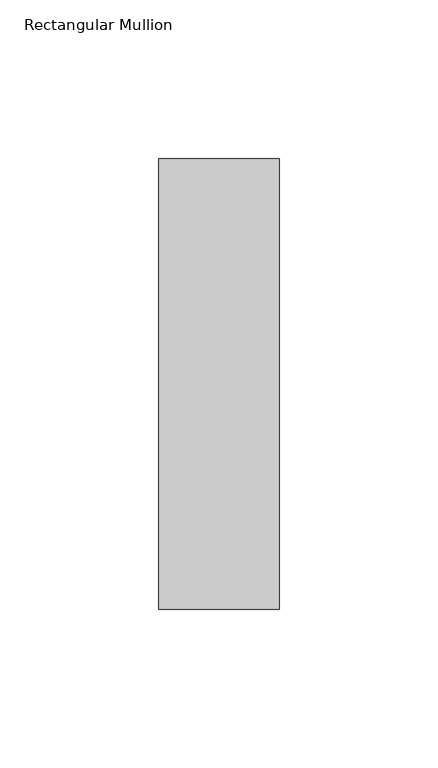
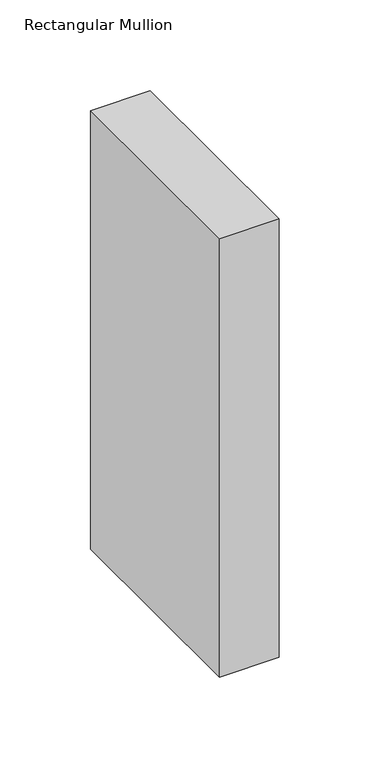
"""IFC4 building model written with IfcOpenShell, lengths in millimetres: member geometry, Rectangular Mullion : NLRS_21_CWM_hsb-regel 38x142_gen_rsf."""

from ifc_helpers import new_model, si_unit, frame, origin, place, context, project, spatial, polyline, outline, extrude, source, transform, mapped, element, save


def rectangular_mullion_e102e68a(model_context):
    return source(origin(), model_context, "Body", "SweptSolid", [
        extrude(outline(polyline([(-38.0, -71.0), (-38.0, 71.0), (0.0, 71.0), (0.0, -71.0), (-38.0, -71.0)])), frame((0.0, 0.0, -295.0), z_axis=(0.0, 0.0, 1.0), x_axis=(1.0, 0.0, 0.0)), (0.0, 0.0, 1.0), 295.0),
    ])


if __name__ == "__main__":
    model = new_model("IFC4")
    model_context = context("Model", 3, world=origin())
    ifc_project = project(units=[si_unit("LENGTHUNIT", "METRE", prefix="MILLI")], contexts=[model_context])
    site = spatial("IfcSite", under=ifc_project)
    building = spatial("IfcBuilding", under=site)
    placement = place(None, origin())
    rectangular_mullion_shape = rectangular_mullion_e102e68a(model_context)
    element("IfcMember", 1, ObjectType="Rectangular Mullion : NLRS_21_CWM_hsb-regel 38x142_gen_rsf", at=placement, inside=building, context=model_context, shape_type="MappedRepresentation", body=[
        mapped(rectangular_mullion_shape, transform((0.0, 0.0, 0.0), x_axis=(1.0, 0.0, 0.0), y_axis=(0.0, 1.0, 0.0), z_axis=(0.0, 0.0, 1.0))),
    ])
    save(model, "model.ifc")

# Revit data of these elements
# Type "Rectangular Mullion : NLRS_21_CWM_hsb-regel 38x142_gen_rsf"
#   Export Type to IFC As = "IfcWall"
#   Type IfcGUID = "07M7mRoiH1CR8m_RSKIwpF"
#   Assembly Code = "21.10"
#   built-in parameter 1007322 = 0.465879 (stored number, unit not read)
#   built-in parameter 1007321 = 0.062336 (stored number, unit not read)
#   built-in parameter 1007320 = 0.062336 (stored number, unit not read)
# Element 1 (IfcMember, "Rectangular Mullion : NLRS_21_CWM_hsb-regel 38x142_gen_rsf")
#   Materials on its faces: "NLRS_i2_hout naaldhout vuren_gen_rsf"
# Materials
#   "NLRS_i2_hout naaldhout vuren_gen_rsf": class "I - Hout", colour RGB 234 199 147, transparency 0, Keynote = "i2", Manufacturer = "Revit Standards Foundation", URL = "www.revitstandards.org", Description = "hout vuren", Cost = 0
